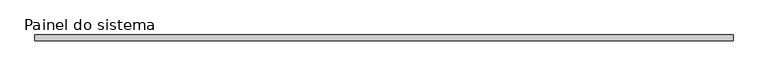
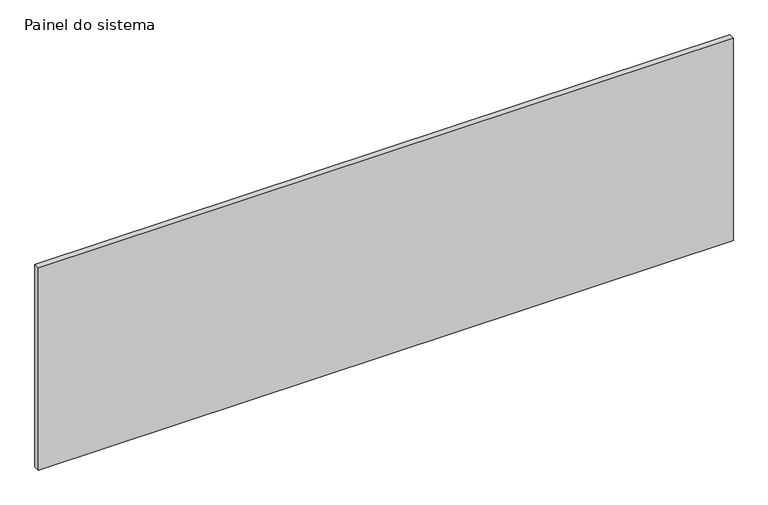
"""IFC4 building model written with IfcOpenShell, lengths in millimetres: plate geometry, Painel do sistema : Envidraçado."""

from ifc_helpers import new_model, si_unit, origin, origin_with_axes, place, context, project, spatial, polyline, outline, extrude, source, transform, mapped, element, save


def painel_do_sistema_36c24d4a(model_context):
    return source(origin(), model_context, "Body", "SweptSolid", [
        extrude(outline(polyline([(1462.5000336, -49.5), (-1462.5000336, -49.5), (-1462.5000336, -24.5), (1462.5000336, -24.5), (1462.5000336, -49.5)])), origin_with_axes(), (0.0, 0.0, 1.0), 900.0),
    ])


if __name__ == "__main__":
    model = new_model("IFC4")
    model_context = context("Model", 3, world=origin())
    ifc_project = project(units=[si_unit("LENGTHUNIT", "METRE", prefix="MILLI")], contexts=[model_context])
    site = spatial("IfcSite", under=ifc_project)
    building = spatial("IfcBuilding", under=site)
    placement = place(None, origin())
    painel_do_sistema_shape = painel_do_sistema_36c24d4a(model_context)
    element("IfcPlate", 1, ObjectType="Painel do sistema : Envidraçado", at=placement, inside=building, context=model_context, shape_type="MappedRepresentation", body=[
        mapped(painel_do_sistema_shape, transform((0.0, 0.0, 0.0), x_axis=(1.0, 0.0, 0.0), y_axis=(0.0, 1.0, 0.0), z_axis=(0.0, 0.0, 1.0))),
    ])
    save(model, "model.ifc")

# Revit data of these elements
# Type "Painel do sistema : Envidraçado"
#   Construction Type Id = "GSP4R"
#   Analytic Construction = "Vidraça única Pilkington 1/8 pol"
#   Visual Light Transmittance = 0.9
#   Solar Heat Gain Coefficient = 0.86
#   Heat Transfer Coefficient (U) = 6.7069 W/(m²·K)
# Element 1 (IfcPlate, "Painel do sistema : Envidraçado")
#   Materials on its faces: "Vidro"
# Materials
#   "Vidro": class "Vidro", colour RGB 0 128 192, transparency 0.9, Description = "Vidro de sílica", Cost = 0
